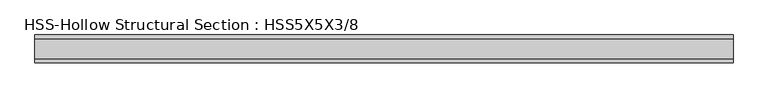
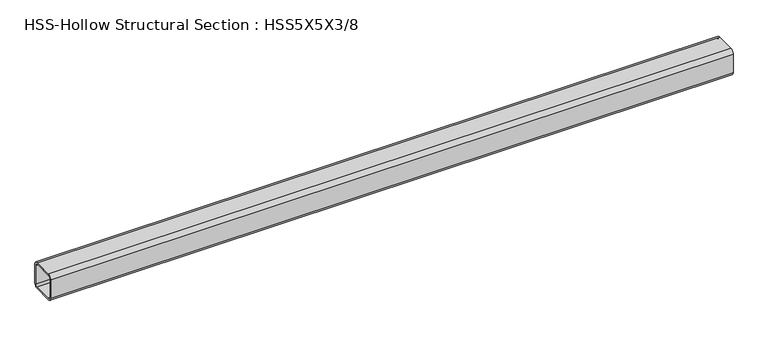
"""IFC4 building model written with IfcOpenShell, lengths in millimetres: member geometry, HSS-Hollow Structural Section : HSS5X5X3/8."""

from ifc_helpers import new_model, si_unit, point, frame, frame_2d, origin, place, context, project, spatial, polyline, circle_curve, trimmed, segment, composite_curve, outline, extrude, source, transform, mapped, element, save


def hss_hollow_structural_section_hss5x5x3_8_04333b48(model_context):
    return source(origin(), model_context, "Body", "SweptSolid", [
        extrude(outline(composite_curve([segment(polyline([(63.5, 45.7708), (63.5, -45.7708)]), True, "CONTINUOUS"), segment(trimmed(circle_curve(frame_2d((45.7708, -45.7708)), 17.7292), [point((63.5, -45.7708))], [point((45.7708, -63.5))], False, "CARTESIAN"), True, "CONTINUOUS"), segment(polyline([(45.7708, -63.5), (-45.7708, -63.5)]), True, "CONTINUOUS"), segment(trimmed(circle_curve(frame_2d((-45.7708, -45.7708)), 17.7292), [point((-45.7708, -63.5))], [point((-63.5, -45.7708))], False, "CARTESIAN"), True, "CONTINUOUS"), segment(polyline([(-63.5, -45.7708), (-63.5, 45.7708)]), True, "CONTINUOUS"), segment(trimmed(circle_curve(frame_2d((-45.7708, 45.7708)), 17.7292), [point((-63.5, 45.7708))], [point((-45.7708, 63.5))], False, "CARTESIAN"), True, "CONTINUOUS"), segment(polyline([(-45.7708, 63.5), (45.7708, 63.5)]), True, "CONTINUOUS"), segment(trimmed(circle_curve(frame_2d((45.7708, 45.7708)), 17.7292), [point((45.7708, 63.5))], [point((63.5, 45.7708))], False, "CARTESIAN"), True, "CONTINUOUS")], self_intersect=False), holes=[composite_curve([segment(trimmed(circle_curve(frame_2d((-45.7708, 45.7708)), 8.8646), [point((-45.7708, 54.6354))], [point((-54.6354, 45.7708))], True, "CARTESIAN"), True, "CONTINUOUS"), segment(polyline([(-54.6354, 45.7708), (-54.6354, -45.7708)]), True, "CONTINUOUS"), segment(trimmed(circle_curve(frame_2d((-45.7708, -45.7708)), 8.8646), [point((-54.6354, -45.7708))], [point((-45.7708, -54.6354))], True, "CARTESIAN"), True, "CONTINUOUS"), segment(polyline([(-45.7708, -54.6354), (45.7708, -54.6354)]), True, "CONTINUOUS"), segment(trimmed(circle_curve(frame_2d((45.7708, -45.7708)), 8.8646), [point((45.7708, -54.6354))], [point((54.6354, -45.7708))], True, "CARTESIAN"), True, "CONTINUOUS"), segment(polyline([(54.6354, -45.7708), (54.6354, 45.7708)]), True, "CONTINUOUS"), segment(trimmed(circle_curve(frame_2d((45.7708, 45.7708)), 8.8646), [point((54.6354, 45.7708))], [point((45.7708, 54.6354))], True, "CARTESIAN"), True, "CONTINUOUS"), segment(polyline([(45.7708, 54.6354), (-45.7708, 54.6354)]), True, "CONTINUOUS")], self_intersect=False)]), frame((-1590.4198661, 0.0, 0.0), z_axis=(1.0, 0.0, 0.0), x_axis=(0.0, 1.0, 0.0)), (0.0, 0.0, 1.0), 3180.8397321),
    ])


if __name__ == "__main__":
    model = new_model("IFC4")
    model_context = context("Model", 3, world=origin())
    ifc_project = project(units=[si_unit("LENGTHUNIT", "METRE", prefix="MILLI")], contexts=[model_context])
    site = spatial("IfcSite", under=ifc_project)
    building = spatial("IfcBuilding", under=site)
    placement = place(None, origin())
    hss_hollow_structural_section_hss5x5x3_8_shape = hss_hollow_structural_section_hss5x5x3_8_04333b48(model_context)
    element("IfcMember", 1, ObjectType="HSS-Hollow Structural Section : HSS5X5X3/8", at=placement, inside=building, context=model_context, shape_type="MappedRepresentation", body=[
        mapped(hss_hollow_structural_section_hss5x5x3_8_shape, transform((0.0, 0.0, 0.0), x_axis=(1.0, 0.0, 0.0), y_axis=(0.0, 1.0, 0.0), z_axis=(0.0, 0.0, 1.0))),
    ])
    save(model, "model.ifc")

# Revit data of these elements
# Type "HSS-Hollow Structural Section : HSS5X5X3/8"
#   Assembly Code = "B10"
#   Shape = "Square"
#   W = 22.3
#   Ht = 0' - 5"
#   Length [instance default] = 5' - 0"
#   b = 0' - 5"
#   kr = 0' - 0.698"
#   t = 0' - 0.349"
#   A = 0.0429167 SF
#   Structural Material [instance default] = Steel ASTM A500, Grade B, Rectangular and Square
# Element 1 (IfcMember, "HSS-Hollow Structural Section : HSS5X5X3/8")
#   Materials on its faces: "Steel ASTM A500, Grade B, Rectangular and Square"
# Materials
#   "Steel ASTM A500, Grade B, Rectangular and Square": class "Metal", colour RGB 199 199 199, transparency 0, Description = "Carbon steel", Cost = 0
